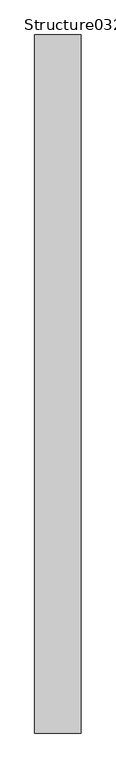
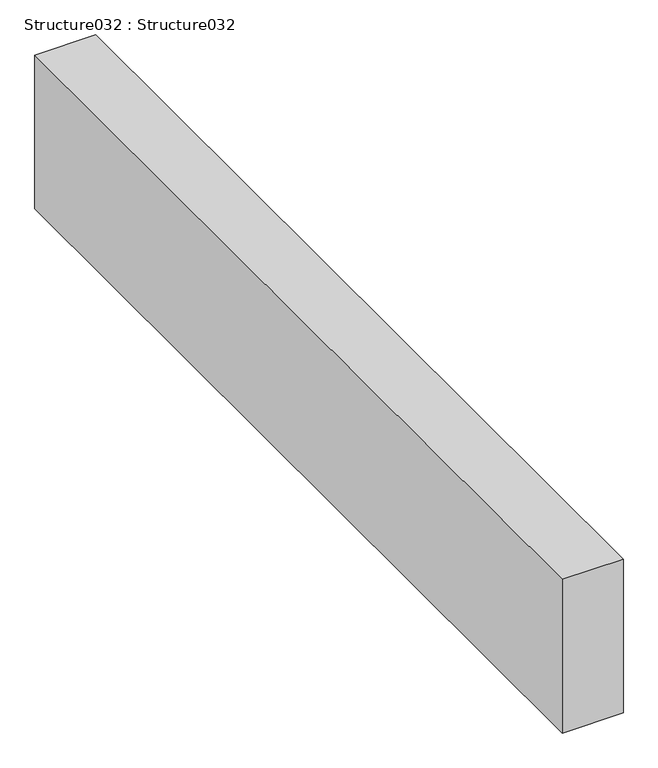
"""IFC4 building model written with IfcOpenShell, lengths in millimetres: proxy geometry, Structure032 : Structure032."""

import ifcopenshell
import ifcopenshell.guid

model = None  # the IFC model being written
_history = None  # IfcOwnerHistory: only IFC2X3 demands one
_inside = {}  # id of a spatial element -> (the spatial element, [elements in it])
_under = {}  # id of a project, library or spatial element -> (it, [spatial elements below it])
_declared = {}  # id of a project -> (the project, [libraries it declares])
_typed = {}  # id of a type object -> (the type object, [elements of that type])
_made_of = {}  # id of a material, layer set ... -> (it, [elements and type objects made of it])


def new_model(schema):
    """Start an empty IFC model of exactly this schema.

    Asked for "IFC4X3", IfcOpenShell would pick the latest addendum, in which some entities
    have other attributes; the version numbers below select the first issue.
    IFC2X3 requires an IfcOwnerHistory on every rooted entity: one is made here for all.
    """
    global model, _history
    if schema == "IFC4X3":
        model = ifcopenshell.file(schema_version=(4, 3, 0, 0))
    else:
        model = ifcopenshell.file(schema=schema)
    _inside.clear()
    _under.clear()
    _declared.clear()
    _typed.clear()
    _made_of.clear()
    _history = None
    if model.schema == "IFC2X3":
        org = make("IfcOrganization", Name="unknown")
        user = make(
            "IfcPersonAndOrganization",
            ThePerson=make("IfcPerson", FamilyName="unknown"),
            TheOrganization=org,
        )
        app = make(
            "IfcApplication",
            ApplicationDeveloper=org,
            Version="unknown",
            ApplicationFullName="unknown",
            ApplicationIdentifier="unknown",
        )
        _history = make(
            "IfcOwnerHistory",
            OwningUser=user,
            OwningApplication=app,
            ChangeAction="ADDED",
            CreationDate=0,
        )
    return model


def make(cls, **values):
    """One entity of the class cls with the attributes given. An attribute that is None is left unset."""
    return model.create_entity(
        cls, **{name: value for name, value in values.items() if value is not None}
    )


def rooted(cls, **values):
    """An entity with a GlobalId (a new one), such as an element, a storey or a relation."""
    return make(cls, GlobalId=ifcopenshell.guid.new(), OwnerHistory=_history, **values)


def si_unit(unit_type, name, prefix=None):
    """IfcSIUnit, for example si_unit("LENGTHUNIT", "METRE", prefix="MILLI")."""
    return make("IfcSIUnit", UnitType=unit_type, Prefix=prefix, Name=name)


def assignment(units):
    """IfcUnitAssignment: the units of a project."""
    return None if units is None else make("IfcUnitAssignment", Units=units)


def point(xyz):
    """IfcCartesianPoint."""
    return None if xyz is None else make("IfcCartesianPoint", Coordinates=xyz)


def direction(xyz):
    """IfcDirection."""
    return None if xyz is None else make("IfcDirection", DirectionRatios=xyz)


def frame(location, z_axis=None, x_axis=None):
    """IfcAxis2Placement3D, a coordinate frame: its origin and axes. An axis left out is left unset."""
    return make(
        "IfcAxis2Placement3D",
        Location=point(location),
        Axis=direction(z_axis),
        RefDirection=direction(x_axis),
    )


def origin():
    """The frame at (0, 0, 0) with its axes left unset."""
    return frame((0.0, 0.0, 0.0))


def place(relative_to, where):
    """IfcLocalPlacement: puts the frame where relative to a parent placement (None: the world)."""
    return make(
        "IfcLocalPlacement", PlacementRelTo=relative_to, RelativePlacement=where
    )


def context(
    kind, dimensions, precision=None, world=None, true_north=None, identifier=None
):
    """IfcGeometricRepresentationContext, for example the 3D "Model" context."""
    return make(
        "IfcGeometricRepresentationContext",
        ContextIdentifier=identifier,
        ContextType=kind,
        CoordinateSpaceDimension=dimensions,
        Precision=precision,
        WorldCoordinateSystem=world,
        TrueNorth=true_north,
    )


def project(units=None, contexts=None):
    """IfcProject with its units and contexts."""
    return rooted(
        "IfcProject",
        Name="project",
        RepresentationContexts=contexts,
        UnitsInContext=assignment(units),
    )


def spatial(cls, under=None, at=None, **own):
    """A site, building, storey or space (cls), placed at a placement, below another one or the project."""
    s = rooted(cls, ObjectPlacement=at, **own)
    if under is not None:
        _under.setdefault(under.id(), (under, []))[1].append(s)
    return s


def polyline(points):
    """IfcPolyline through the points."""
    return make("IfcPolyline", Points=[point(p) for p in points])


def outline(outer, holes=None, kind="AREA"):
    """IfcArbitraryClosedProfileDef: a profile drawn as a closed curve; with holes, ...WithVoids."""
    if holes is None:
        return make("IfcArbitraryClosedProfileDef", ProfileType=kind, OuterCurve=outer)
    return make(
        "IfcArbitraryProfileDefWithVoids",
        ProfileType=kind,
        OuterCurve=outer,
        InnerCurves=holes,
    )


def extrude(swept, where, along, depth):
    """IfcExtrudedAreaSolid: the profile swept, set in the frame where, extruded along a direction by depth."""
    return make(
        "IfcExtrudedAreaSolid",
        SweptArea=swept,
        Position=where,
        ExtrudedDirection=direction(along),
        Depth=depth,
    )


def shape(context_of_items, identifier, shape_type, items):
    """IfcShapeRepresentation: the items that make up one representation, for example the "Body"."""
    return make(
        "IfcShapeRepresentation",
        ContextOfItems=context_of_items,
        RepresentationIdentifier=identifier,
        RepresentationType=shape_type,
        Items=items,
    )


def source(mapping_origin, context_of_items, identifier, shape_type, items):
    """IfcRepresentationMap: a shape defined once, which mapped items show again and again."""
    return make(
        "IfcRepresentationMap",
        MappingOrigin=mapping_origin,
        MappedRepresentation=shape(context_of_items, identifier, shape_type, items),
    )


def transform(
    local_origin,
    x_axis=None,
    y_axis=None,
    z_axis=None,
    scale=None,
    scale2=None,
    scale3=None,
    uniform=True,
):
    """IfcCartesianTransformationOperator3D, or its non-uniform kind. x_axis, y_axis, z_axis: its Axis1, 2, 3."""
    if uniform:
        return make(
            "IfcCartesianTransformationOperator3D",
            Axis1=direction(x_axis),
            Axis2=direction(y_axis),
            LocalOrigin=point(local_origin),
            Scale=scale,
            Axis3=direction(z_axis),
        )
    return make(
        "IfcCartesianTransformationOperator3DnonUniform",
        Axis1=direction(x_axis),
        Axis2=direction(y_axis),
        LocalOrigin=point(local_origin),
        Scale=scale,
        Axis3=direction(z_axis),
        Scale2=scale2,
        Scale3=scale3,
    )


def mapped(mapping_source, mapping_target):
    """IfcMappedItem: shows the shape of a source again, moved by a transform."""
    return make(
        "IfcMappedItem", MappingSource=mapping_source, MappingTarget=mapping_target
    )


def made_of(thing, what):
    """Note that an element or type object is made of a material, layer set ...; save() writes the relation."""
    if what is not None:
        _made_of.setdefault(what.id(), (what, []))[1].append(thing)
    return thing


def element(
    cls,
    number,
    at=None,
    inside=None,
    cuts=None,
    type_object=None,
    material=None,
    context=None,
    identifier="Body",
    shape_type=None,
    held_by="IfcProductDefinitionShape",
    body=None,
    shapes=None,
    **own,
):
    """One element of the class cls, such as IfcWall. Its Tag is "e" and its number.

    at: its placement. inside: the storey or other place that contains it. cuts: it is an
    opening in that element (IfcRelVoidsElement). A single representation is given by context,
    identifier, shape_type and body (its items); several are given by shapes. held_by: the class
    of the entity that holds the representations. save() writes the other relations.
    """
    e = rooted(cls, Tag="e%d" % number, ObjectPlacement=at, **own)
    if body is not None:
        shapes = [shape(context, identifier, shape_type, body)]
    if shapes is not None:
        e.Representation = make(held_by, Representations=shapes)
    if inside is not None:
        _inside.setdefault(inside.id(), (inside, []))[1].append(e)
    if cuts is not None:
        rooted(
            "IfcRelVoidsElement", RelatingBuildingElement=cuts, RelatedOpeningElement=e
        )
    if type_object is not None:
        _typed.setdefault(type_object.id(), (type_object, []))[1].append(e)
    return made_of(e, material)


def aggregate(whole, parts):
    """IfcRelAggregates: a whole, such as a stair, and the parts it consists of."""
    return rooted("IfcRelAggregates", RelatingObject=whole, RelatedObjects=parts)


def save(model, path):
    """Write the relations noted so far, then the file.

    IfcRelAggregates (storeys below a building ...), IfcRelContainedInSpatialStructure (elements
    in a storey), IfcRelDefinesByType, IfcRelAssociatesMaterial and IfcRelDeclares: one each for
    every whole, place, type object, material and project.
    """
    for whole, parts in _under.values():
        aggregate(whole, parts)
    for where, things in _inside.values():
        rooted(
            "IfcRelContainedInSpatialStructure",
            RelatedElements=things,
            RelatingStructure=where,
        )
    for kind, things in _typed.values():
        rooted("IfcRelDefinesByType", RelatedObjects=things, RelatingType=kind)
    for what, things in _made_of.values():
        rooted("IfcRelAssociatesMaterial", RelatedObjects=things, RelatingMaterial=what)
    for by, libraries in _declared.values():
        rooted("IfcRelDeclares", RelatingContext=by, RelatedDefinitions=libraries)
    model.write(path)


def structure032_structure032_4a1b2fea(model_context):
    return source(origin(), model_context, "Body", "SweptSolid", [
        extrude(outline(polyline([(-4806.5557607, 7982.1531721), (-4939.9057607, 7982.1531721), (-4939.9057607, 9982.1531721), (-4806.5557607, 9982.1531721), (-4806.5557607, 7982.1531721)])), frame((0.0, 0.0, 43055.5617235), z_axis=(0.0, 0.0, 1.0), x_axis=(1.0, 0.0, 0.0)), (0.0, 0.0, 1.0), 355.6),
    ])


if __name__ == "__main__":
    model = new_model("IFC4")
    model_context = context("Model", 3, world=origin())
    ifc_project = project(units=[si_unit("LENGTHUNIT", "METRE", prefix="MILLI")], contexts=[model_context])
    site = spatial("IfcSite", under=ifc_project)
    building = spatial("IfcBuilding", under=site)
    placement = place(None, origin())
    structure032_structure032_shape = structure032_structure032_4a1b2fea(model_context)
    element("IfcBuildingElementProxy", 1, Name="Structure032 : Structure032", ObjectType="Structure032 : Structure032", at=placement, inside=building, context=model_context, shape_type="MappedRepresentation", body=[
        mapped(structure032_structure032_shape, transform((0.0, 0.0, 0.0), x_axis=(1.0, 0.0, 0.0), y_axis=(0.0, 1.0, 0.0), z_axis=(0.0, 0.0, 1.0))),
    ])
    save(model, "model.ifc")

# Revit data of these elements
# Type "Structure032 : Structure032"
#   NameOverride = "Structure032"
# Element 1 (IfcBuildingElementProxy, "Structure032 : Structure032")
#   Materials on its faces: "STRUCTURAL MEMBER (SEE STRUCTURAL DWGS)"
# Materials
#   "STRUCTURAL MEMBER (SEE STRUCTURAL DWGS)": class "Unassigned", colour RGB 176 134 95, transparency 0, Cost = 0
